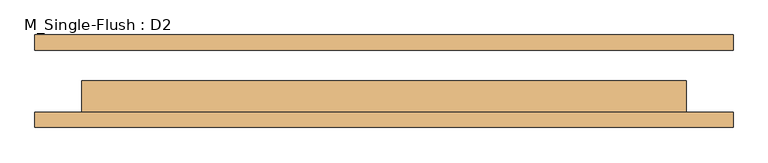
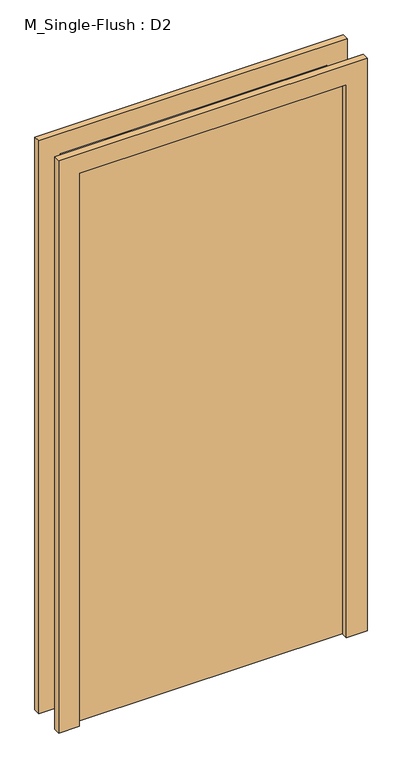
"""IFC4 building model written with IfcOpenShell, lengths in millimetres: door geometry, M_Single-Flush : D2."""

import ifcopenshell
import ifcopenshell.guid

model = None  # the IFC model being written
_history = None  # IfcOwnerHistory: only IFC2X3 demands one
_inside = {}  # id of a spatial element -> (the spatial element, [elements in it])
_under = {}  # id of a project, library or spatial element -> (it, [spatial elements below it])
_declared = {}  # id of a project -> (the project, [libraries it declares])
_typed = {}  # id of a type object -> (the type object, [elements of that type])
_made_of = {}  # id of a material, layer set ... -> (it, [elements and type objects made of it])


def new_model(schema):
    """Start an empty IFC model of exactly this schema.

    Asked for "IFC4X3", IfcOpenShell would pick the latest addendum, in which some entities
    have other attributes; the version numbers below select the first issue.
    IFC2X3 requires an IfcOwnerHistory on every rooted entity: one is made here for all.
    """
    global model, _history
    if schema == "IFC4X3":
        model = ifcopenshell.file(schema_version=(4, 3, 0, 0))
    else:
        model = ifcopenshell.file(schema=schema)
    _inside.clear()
    _under.clear()
    _declared.clear()
    _typed.clear()
    _made_of.clear()
    _history = None
    if model.schema == "IFC2X3":
        org = make("IfcOrganization", Name="unknown")
        user = make(
            "IfcPersonAndOrganization",
            ThePerson=make("IfcPerson", FamilyName="unknown"),
            TheOrganization=org,
        )
        app = make(
            "IfcApplication",
            ApplicationDeveloper=org,
            Version="unknown",
            ApplicationFullName="unknown",
            ApplicationIdentifier="unknown",
        )
        _history = make(
            "IfcOwnerHistory",
            OwningUser=user,
            OwningApplication=app,
            ChangeAction="ADDED",
            CreationDate=0,
        )
    return model


def make(cls, **values):
    """One entity of the class cls with the attributes given. An attribute that is None is left unset."""
    return model.create_entity(
        cls, **{name: value for name, value in values.items() if value is not None}
    )


def rooted(cls, **values):
    """An entity with a GlobalId (a new one), such as an element, a storey or a relation."""
    return make(cls, GlobalId=ifcopenshell.guid.new(), OwnerHistory=_history, **values)


def si_unit(unit_type, name, prefix=None):
    """IfcSIUnit, for example si_unit("LENGTHUNIT", "METRE", prefix="MILLI")."""
    return make("IfcSIUnit", UnitType=unit_type, Prefix=prefix, Name=name)


def assignment(units):
    """IfcUnitAssignment: the units of a project."""
    return None if units is None else make("IfcUnitAssignment", Units=units)


def point(xyz):
    """IfcCartesianPoint."""
    return None if xyz is None else make("IfcCartesianPoint", Coordinates=xyz)


def direction(xyz):
    """IfcDirection."""
    return None if xyz is None else make("IfcDirection", DirectionRatios=xyz)


def frame(location, z_axis=None, x_axis=None):
    """IfcAxis2Placement3D, a coordinate frame: its origin and axes. An axis left out is left unset."""
    return make(
        "IfcAxis2Placement3D",
        Location=point(location),
        Axis=direction(z_axis),
        RefDirection=direction(x_axis),
    )


def origin():
    """The frame at (0, 0, 0) with its axes left unset."""
    return frame((0.0, 0.0, 0.0))


def origin_with_axes():
    """The frame at (0, 0, 0) with the z axis (0, 0, 1) and the x axis (1, 0, 0) written out."""
    return frame((0.0, 0.0, 0.0), z_axis=(0.0, 0.0, 1.0), x_axis=(1.0, 0.0, 0.0))


def place(relative_to, where):
    """IfcLocalPlacement: puts the frame where relative to a parent placement (None: the world)."""
    return make(
        "IfcLocalPlacement", PlacementRelTo=relative_to, RelativePlacement=where
    )


def context(
    kind, dimensions, precision=None, world=None, true_north=None, identifier=None
):
    """IfcGeometricRepresentationContext, for example the 3D "Model" context."""
    return make(
        "IfcGeometricRepresentationContext",
        ContextIdentifier=identifier,
        ContextType=kind,
        CoordinateSpaceDimension=dimensions,
        Precision=precision,
        WorldCoordinateSystem=world,
        TrueNorth=true_north,
    )


def project(units=None, contexts=None):
    """IfcProject with its units and contexts."""
    return rooted(
        "IfcProject",
        Name="project",
        RepresentationContexts=contexts,
        UnitsInContext=assignment(units),
    )


def spatial(cls, under=None, at=None, **own):
    """A site, building, storey or space (cls), placed at a placement, below another one or the project."""
    s = rooted(cls, ObjectPlacement=at, **own)
    if under is not None:
        _under.setdefault(under.id(), (under, []))[1].append(s)
    return s


def polyline(points):
    """IfcPolyline through the points."""
    return make("IfcPolyline", Points=[point(p) for p in points])


def outline(outer, holes=None, kind="AREA"):
    """IfcArbitraryClosedProfileDef: a profile drawn as a closed curve; with holes, ...WithVoids."""
    if holes is None:
        return make("IfcArbitraryClosedProfileDef", ProfileType=kind, OuterCurve=outer)
    return make(
        "IfcArbitraryProfileDefWithVoids",
        ProfileType=kind,
        OuterCurve=outer,
        InnerCurves=holes,
    )


def extrude(swept, where, along, depth):
    """IfcExtrudedAreaSolid: the profile swept, set in the frame where, extruded along a direction by depth."""
    return make(
        "IfcExtrudedAreaSolid",
        SweptArea=swept,
        Position=where,
        ExtrudedDirection=direction(along),
        Depth=depth,
    )


def shape(context_of_items, identifier, shape_type, items):
    """IfcShapeRepresentation: the items that make up one representation, for example the "Body"."""
    return make(
        "IfcShapeRepresentation",
        ContextOfItems=context_of_items,
        RepresentationIdentifier=identifier,
        RepresentationType=shape_type,
        Items=items,
    )


def source(mapping_origin, context_of_items, identifier, shape_type, items):
    """IfcRepresentationMap: a shape defined once, which mapped items show again and again."""
    return make(
        "IfcRepresentationMap",
        MappingOrigin=mapping_origin,
        MappedRepresentation=shape(context_of_items, identifier, shape_type, items),
    )


def transform(
    local_origin,
    x_axis=None,
    y_axis=None,
    z_axis=None,
    scale=None,
    scale2=None,
    scale3=None,
    uniform=True,
):
    """IfcCartesianTransformationOperator3D, or its non-uniform kind. x_axis, y_axis, z_axis: its Axis1, 2, 3."""
    if uniform:
        return make(
            "IfcCartesianTransformationOperator3D",
            Axis1=direction(x_axis),
            Axis2=direction(y_axis),
            LocalOrigin=point(local_origin),
            Scale=scale,
            Axis3=direction(z_axis),
        )
    return make(
        "IfcCartesianTransformationOperator3DnonUniform",
        Axis1=direction(x_axis),
        Axis2=direction(y_axis),
        LocalOrigin=point(local_origin),
        Scale=scale,
        Axis3=direction(z_axis),
        Scale2=scale2,
        Scale3=scale3,
    )


def mapped(mapping_source, mapping_target):
    """IfcMappedItem: shows the shape of a source again, moved by a transform."""
    return make(
        "IfcMappedItem", MappingSource=mapping_source, MappingTarget=mapping_target
    )


def made_of(thing, what):
    """Note that an element or type object is made of a material, layer set ...; save() writes the relation."""
    if what is not None:
        _made_of.setdefault(what.id(), (what, []))[1].append(thing)
    return thing


def element(
    cls,
    number,
    at=None,
    inside=None,
    cuts=None,
    type_object=None,
    material=None,
    context=None,
    identifier="Body",
    shape_type=None,
    held_by="IfcProductDefinitionShape",
    body=None,
    shapes=None,
    **own,
):
    """One element of the class cls, such as IfcWall. Its Tag is "e" and its number.

    at: its placement. inside: the storey or other place that contains it. cuts: it is an
    opening in that element (IfcRelVoidsElement). A single representation is given by context,
    identifier, shape_type and body (its items); several are given by shapes. held_by: the class
    of the entity that holds the representations. save() writes the other relations.
    """
    e = rooted(cls, Tag="e%d" % number, ObjectPlacement=at, **own)
    if body is not None:
        shapes = [shape(context, identifier, shape_type, body)]
    if shapes is not None:
        e.Representation = make(held_by, Representations=shapes)
    if inside is not None:
        _inside.setdefault(inside.id(), (inside, []))[1].append(e)
    if cuts is not None:
        rooted(
            "IfcRelVoidsElement", RelatingBuildingElement=cuts, RelatedOpeningElement=e
        )
    if type_object is not None:
        _typed.setdefault(type_object.id(), (type_object, []))[1].append(e)
    return made_of(e, material)


def aggregate(whole, parts):
    """IfcRelAggregates: a whole, such as a stair, and the parts it consists of."""
    return rooted("IfcRelAggregates", RelatingObject=whole, RelatedObjects=parts)


def save(model, path):
    """Write the relations noted so far, then the file.

    IfcRelAggregates (storeys below a building ...), IfcRelContainedInSpatialStructure (elements
    in a storey), IfcRelDefinesByType, IfcRelAssociatesMaterial and IfcRelDeclares: one each for
    every whole, place, type object, material and project.
    """
    for whole, parts in _under.values():
        aggregate(whole, parts)
    for where, things in _inside.values():
        rooted(
            "IfcRelContainedInSpatialStructure",
            RelatedElements=things,
            RelatingStructure=where,
        )
    for kind, things in _typed.values():
        rooted("IfcRelDefinesByType", RelatedObjects=things, RelatingType=kind)
    for what, things in _made_of.values():
        rooted("IfcRelAssociatesMaterial", RelatedObjects=things, RelatingMaterial=what)
    for by, libraries in _declared.values():
        rooted("IfcRelDeclares", RelatingContext=by, RelatedDefinitions=libraries)
    model.write(path)


def m_single_flush_d2_462e7c1d(model_context):
    return source(origin(), model_context, "Body", "SweptSolid", [
        extrude(outline(polyline([(2221.0, -566.0), (0.0, -566.0), (0.0, -490.0), (2145.0, -490.0), (2145.0, 490.0), (0.0, 490.0), (0.0, 566.0), (2221.0, 566.0), (2221.0, -566.0)])), frame((0.0, -75.0, 0.0), z_axis=(0.0, 1.0, 0.0), x_axis=(0.0, 0.0, 1.0)), (0.0, 0.0, 1.0), 25.0),
        extrude(outline(polyline([(2221.0, 566.0), (2221.0, -566.0), (0.0, -566.0), (0.0, -490.0), (2145.0, -490.0), (2145.0, 490.0), (0.0, 490.0), (0.0, 566.0), (2221.0, 566.0)])), frame((0.0, 50.0, 0.0), z_axis=(0.0, 1.0, 0.0), x_axis=(0.0, 0.0, 1.0)), (0.0, 0.0, 1.0), 25.0),
        extrude(outline(polyline([(490.0, 1.0), (490.0, -50.0), (-490.0, -50.0), (-490.0, 1.0), (490.0, 1.0)])), origin_with_axes(), (0.0, 0.0, 1.0), 2145.0),
    ])


if __name__ == "__main__":
    model = new_model("IFC4")
    model_context = context("Model", 3, world=origin())
    ifc_project = project(units=[si_unit("LENGTHUNIT", "METRE", prefix="MILLI")], contexts=[model_context])
    site = spatial("IfcSite", under=ifc_project)
    building = spatial("IfcBuilding", under=site)
    placement = place(None, origin())
    m_single_flush_d2_shape = m_single_flush_d2_462e7c1d(model_context)
    element("IfcDoor", 1, ObjectType="M_Single-Flush : D2", at=placement, inside=building, context=model_context, shape_type="MappedRepresentation", body=[
        mapped(m_single_flush_d2_shape, transform((0.0, 0.0, 0.0), x_axis=(1.0, 0.0, 0.0), y_axis=(0.0, 1.0, 0.0), z_axis=(0.0, 0.0, 1.0))),
    ])
    save(model, "model.ifc")

# Revit data of these elements
# Type "M_Single-Flush : D2"
#   Type Mark = "23"
#   Thickness = 51 mm
#   Height = 2145 mm
#   Trim Projection Ext = 25 mm
#   Trim Projection Int = 25 mm
#   Trim Width = 76 mm
#   Width = 980 mm
#   Door Material = Door - Panel
#   Frame Material = Door - Frame
#   Function = (empty or 0)
#   Wall Closure = (empty or 0)
# Element 1 (IfcDoor, "M_Single-Flush : D2")
#   Materials on its faces: "Door - Frame", "Door - Panel"
# Materials
#   "Door - Panel": class "Wood", colour RGB 210 159 95, transparency 0
#   "Door - Frame": class "Miscellaneous", colour RGB 118 70 51, transparency 0
